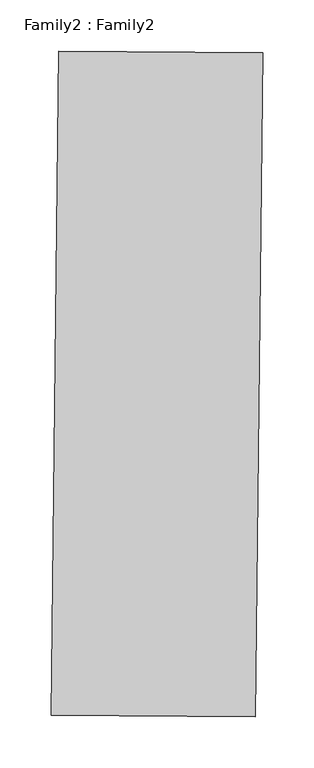
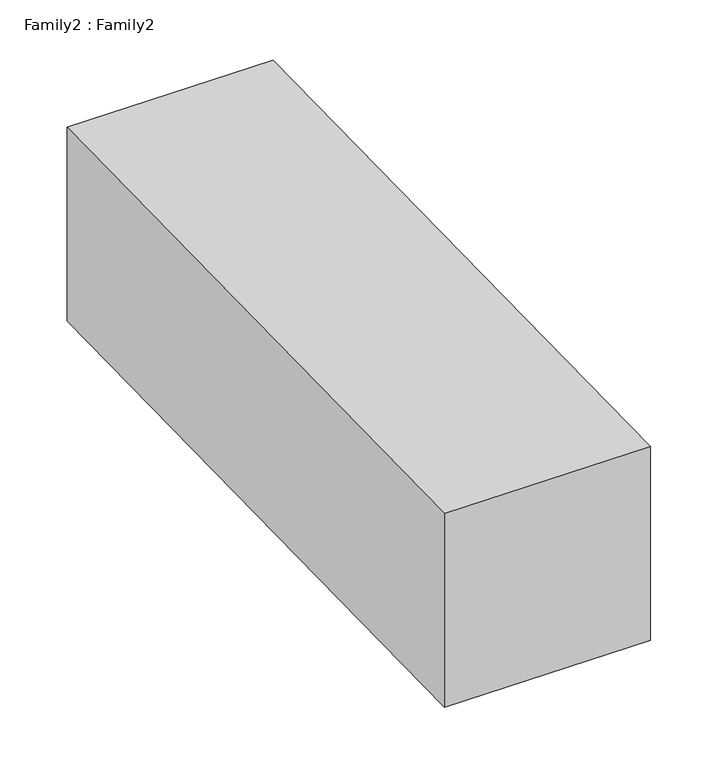
"""IFC4 building model written with IfcOpenShell, lengths in millimetres: proxy geometry, Family2 : Family2."""

import ifcopenshell
import ifcopenshell.guid

model = None  # the IFC model being written
_history = None  # IfcOwnerHistory: only IFC2X3 demands one
_inside = {}  # id of a spatial element -> (the spatial element, [elements in it])
_under = {}  # id of a project, library or spatial element -> (it, [spatial elements below it])
_declared = {}  # id of a project -> (the project, [libraries it declares])
_typed = {}  # id of a type object -> (the type object, [elements of that type])
_made_of = {}  # id of a material, layer set ... -> (it, [elements and type objects made of it])


def new_model(schema):
    """Start an empty IFC model of exactly this schema.

    Asked for "IFC4X3", IfcOpenShell would pick the latest addendum, in which some entities
    have other attributes; the version numbers below select the first issue.
    IFC2X3 requires an IfcOwnerHistory on every rooted entity: one is made here for all.
    """
    global model, _history
    if schema == "IFC4X3":
        model = ifcopenshell.file(schema_version=(4, 3, 0, 0))
    else:
        model = ifcopenshell.file(schema=schema)
    _inside.clear()
    _under.clear()
    _declared.clear()
    _typed.clear()
    _made_of.clear()
    _history = None
    if model.schema == "IFC2X3":
        org = make("IfcOrganization", Name="unknown")
        user = make(
            "IfcPersonAndOrganization",
            ThePerson=make("IfcPerson", FamilyName="unknown"),
            TheOrganization=org,
        )
        app = make(
            "IfcApplication",
            ApplicationDeveloper=org,
            Version="unknown",
            ApplicationFullName="unknown",
            ApplicationIdentifier="unknown",
        )
        _history = make(
            "IfcOwnerHistory",
            OwningUser=user,
            OwningApplication=app,
            ChangeAction="ADDED",
            CreationDate=0,
        )
    return model


def make(cls, **values):
    """One entity of the class cls with the attributes given. An attribute that is None is left unset."""
    return model.create_entity(
        cls, **{name: value for name, value in values.items() if value is not None}
    )


def rooted(cls, **values):
    """An entity with a GlobalId (a new one), such as an element, a storey or a relation."""
    return make(cls, GlobalId=ifcopenshell.guid.new(), OwnerHistory=_history, **values)


def si_unit(unit_type, name, prefix=None):
    """IfcSIUnit, for example si_unit("LENGTHUNIT", "METRE", prefix="MILLI")."""
    return make("IfcSIUnit", UnitType=unit_type, Prefix=prefix, Name=name)


def assignment(units):
    """IfcUnitAssignment: the units of a project."""
    return None if units is None else make("IfcUnitAssignment", Units=units)


def point(xyz):
    """IfcCartesianPoint."""
    return None if xyz is None else make("IfcCartesianPoint", Coordinates=xyz)


def direction(xyz):
    """IfcDirection."""
    return None if xyz is None else make("IfcDirection", DirectionRatios=xyz)


def frame(location, z_axis=None, x_axis=None):
    """IfcAxis2Placement3D, a coordinate frame: its origin and axes. An axis left out is left unset."""
    return make(
        "IfcAxis2Placement3D",
        Location=point(location),
        Axis=direction(z_axis),
        RefDirection=direction(x_axis),
    )


def origin():
    """The frame at (0, 0, 0) with its axes left unset."""
    return frame((0.0, 0.0, 0.0))


def place(relative_to, where):
    """IfcLocalPlacement: puts the frame where relative to a parent placement (None: the world)."""
    return make(
        "IfcLocalPlacement", PlacementRelTo=relative_to, RelativePlacement=where
    )


def context(
    kind, dimensions, precision=None, world=None, true_north=None, identifier=None
):
    """IfcGeometricRepresentationContext, for example the 3D "Model" context."""
    return make(
        "IfcGeometricRepresentationContext",
        ContextIdentifier=identifier,
        ContextType=kind,
        CoordinateSpaceDimension=dimensions,
        Precision=precision,
        WorldCoordinateSystem=world,
        TrueNorth=true_north,
    )


def project(units=None, contexts=None):
    """IfcProject with its units and contexts."""
    return rooted(
        "IfcProject",
        Name="project",
        RepresentationContexts=contexts,
        UnitsInContext=assignment(units),
    )


def spatial(cls, under=None, at=None, **own):
    """A site, building, storey or space (cls), placed at a placement, below another one or the project."""
    s = rooted(cls, ObjectPlacement=at, **own)
    if under is not None:
        _under.setdefault(under.id(), (under, []))[1].append(s)
    return s


def faces_of(points, faces, orient=None, outer=None):
    """IfcFace entities. A face is a list of loops; a loop is a list of indices into points, from 0.

    orient and outer hold one flag for each loop. By default every Orientation is true, the
    first loop of a face is its IfcFaceOuterBound and the others are IfcFaceBound.
    """
    made = []
    for i, loops in enumerate(faces):
        bounds = []
        for j, loop in enumerate(loops):
            is_outer = j == 0 if outer is None else outer[i][j]
            bounds.append(
                make(
                    "IfcFaceOuterBound" if is_outer else "IfcFaceBound",
                    Bound=make("IfcPolyLoop", Polygon=[points[k] for k in loop]),
                    Orientation=True if orient is None else orient[i][j],
                )
            )
        made.append(make("IfcFace", Bounds=bounds))
    return made


def faceted_brep(points, faces, orient=None, outer=None, voids=None):
    """IfcFacetedBrep: a solid bounded by flat faces; with voids (closed shells), ...WithVoids."""
    shared = [point(p) for p in points]
    hull = make("IfcClosedShell", CfsFaces=faces_of(shared, faces, orient, outer))
    if voids is None:
        return make("IfcFacetedBrep", Outer=hull)
    return make(
        "IfcFacetedBrepWithVoids",
        Outer=hull,
        Voids=[
            make(cls, CfsFaces=faces_of(shared, fs, o, b)) for cls, fs, o, b in voids
        ],
    )


def shape(context_of_items, identifier, shape_type, items):
    """IfcShapeRepresentation: the items that make up one representation, for example the "Body"."""
    return make(
        "IfcShapeRepresentation",
        ContextOfItems=context_of_items,
        RepresentationIdentifier=identifier,
        RepresentationType=shape_type,
        Items=items,
    )


def source(mapping_origin, context_of_items, identifier, shape_type, items):
    """IfcRepresentationMap: a shape defined once, which mapped items show again and again."""
    return make(
        "IfcRepresentationMap",
        MappingOrigin=mapping_origin,
        MappedRepresentation=shape(context_of_items, identifier, shape_type, items),
    )


def transform(
    local_origin,
    x_axis=None,
    y_axis=None,
    z_axis=None,
    scale=None,
    scale2=None,
    scale3=None,
    uniform=True,
):
    """IfcCartesianTransformationOperator3D, or its non-uniform kind. x_axis, y_axis, z_axis: its Axis1, 2, 3."""
    if uniform:
        return make(
            "IfcCartesianTransformationOperator3D",
            Axis1=direction(x_axis),
            Axis2=direction(y_axis),
            LocalOrigin=point(local_origin),
            Scale=scale,
            Axis3=direction(z_axis),
        )
    return make(
        "IfcCartesianTransformationOperator3DnonUniform",
        Axis1=direction(x_axis),
        Axis2=direction(y_axis),
        LocalOrigin=point(local_origin),
        Scale=scale,
        Axis3=direction(z_axis),
        Scale2=scale2,
        Scale3=scale3,
    )


def mapped(mapping_source, mapping_target):
    """IfcMappedItem: shows the shape of a source again, moved by a transform."""
    return make(
        "IfcMappedItem", MappingSource=mapping_source, MappingTarget=mapping_target
    )


def made_of(thing, what):
    """Note that an element or type object is made of a material, layer set ...; save() writes the relation."""
    if what is not None:
        _made_of.setdefault(what.id(), (what, []))[1].append(thing)
    return thing


def element(
    cls,
    number,
    at=None,
    inside=None,
    cuts=None,
    type_object=None,
    material=None,
    context=None,
    identifier="Body",
    shape_type=None,
    held_by="IfcProductDefinitionShape",
    body=None,
    shapes=None,
    **own,
):
    """One element of the class cls, such as IfcWall. Its Tag is "e" and its number.

    at: its placement. inside: the storey or other place that contains it. cuts: it is an
    opening in that element (IfcRelVoidsElement). A single representation is given by context,
    identifier, shape_type and body (its items); several are given by shapes. held_by: the class
    of the entity that holds the representations. save() writes the other relations.
    """
    e = rooted(cls, Tag="e%d" % number, ObjectPlacement=at, **own)
    if body is not None:
        shapes = [shape(context, identifier, shape_type, body)]
    if shapes is not None:
        e.Representation = make(held_by, Representations=shapes)
    if inside is not None:
        _inside.setdefault(inside.id(), (inside, []))[1].append(e)
    if cuts is not None:
        rooted(
            "IfcRelVoidsElement", RelatingBuildingElement=cuts, RelatedOpeningElement=e
        )
    if type_object is not None:
        _typed.setdefault(type_object.id(), (type_object, []))[1].append(e)
    return made_of(e, material)


def aggregate(whole, parts):
    """IfcRelAggregates: a whole, such as a stair, and the parts it consists of."""
    return rooted("IfcRelAggregates", RelatingObject=whole, RelatedObjects=parts)


def save(model, path):
    """Write the relations noted so far, then the file.

    IfcRelAggregates (storeys below a building ...), IfcRelContainedInSpatialStructure (elements
    in a storey), IfcRelDefinesByType, IfcRelAssociatesMaterial and IfcRelDeclares: one each for
    every whole, place, type object, material and project.
    """
    for whole, parts in _under.values():
        aggregate(whole, parts)
    for where, things in _inside.values():
        rooted(
            "IfcRelContainedInSpatialStructure",
            RelatedElements=things,
            RelatingStructure=where,
        )
    for kind, things in _typed.values():
        rooted("IfcRelDefinesByType", RelatedObjects=things, RelatingType=kind)
    for what, things in _made_of.values():
        rooted("IfcRelAssociatesMaterial", RelatedObjects=things, RelatingMaterial=what)
    for by, libraries in _declared.values():
        rooted("IfcRelDeclares", RelatingContext=by, RelatedDefinitions=libraries)
    model.write(path)


def family2_family2_428b8be4(model_context):
    return source(origin(), model_context, "Body", "Brep", [
        faceted_brep([(-3947.2904042, -6399.2080776, 1.0945136), (-3947.2904042, -6399.2080776, 201.0945136), (-3939.5523903, -5748.392045, 202.060409), (-3939.5523903, -5748.392045, 2.060409), (-3747.2992142, -6401.0852903, 201.0945136), (-3739.5612004, -5750.2692577, 202.060409), (-3747.2992142, -6401.0852903, 1.0945136), (-3739.5612004, -5750.2692577, 2.060409)], [[[0, 1, 2, 3]], [[1, 4, 5, 2]], [[4, 6, 7, 5]], [[6, 0, 3, 7]], [[3, 2, 5, 7]], [[0, 6, 4, 1]]]),
    ])


if __name__ == "__main__":
    model = new_model("IFC4")
    model_context = context("Model", 3, world=origin())
    ifc_project = project(units=[si_unit("LENGTHUNIT", "METRE", prefix="MILLI")], contexts=[model_context])
    site = spatial("IfcSite", under=ifc_project)
    building = spatial("IfcBuilding", under=site)
    placement = place(None, origin())
    family2_family2_shape = family2_family2_428b8be4(model_context)
    element("IfcBuildingElementProxy", 1, Name="Family2 : Family2", ObjectType="Family2 : Family2", at=placement, inside=building, context=model_context, shape_type="MappedRepresentation", body=[
        mapped(family2_family2_shape, transform((0.0, 0.0, 0.0), x_axis=(1.0, 0.0, 0.0), y_axis=(0.0, 1.0, 0.0), z_axis=(0.0, 0.0, 1.0))),
    ])
    save(model, "model.ifc")

# Revit data of these elements
# Type "Family2 : Family2"
#   Default Elevation = 0
